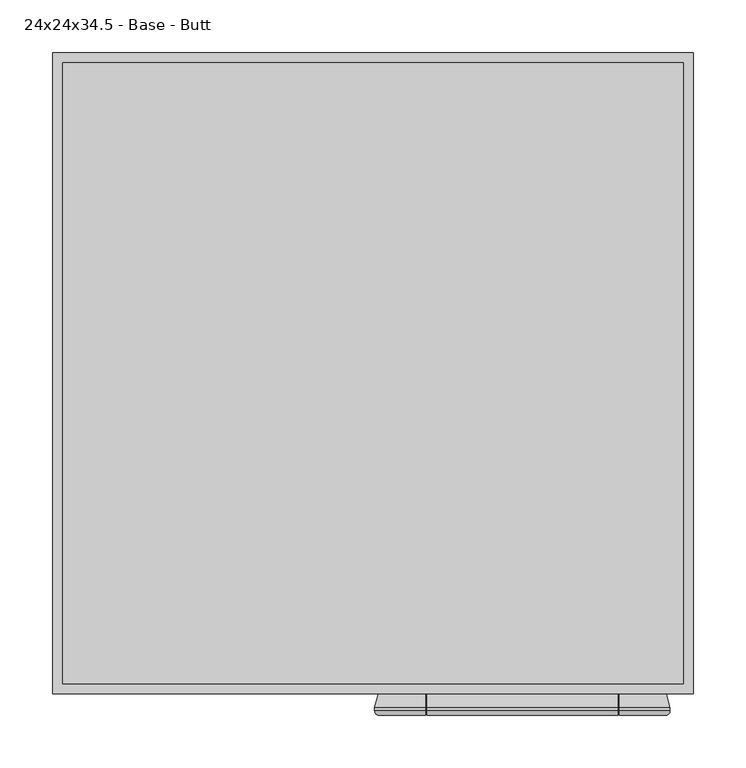
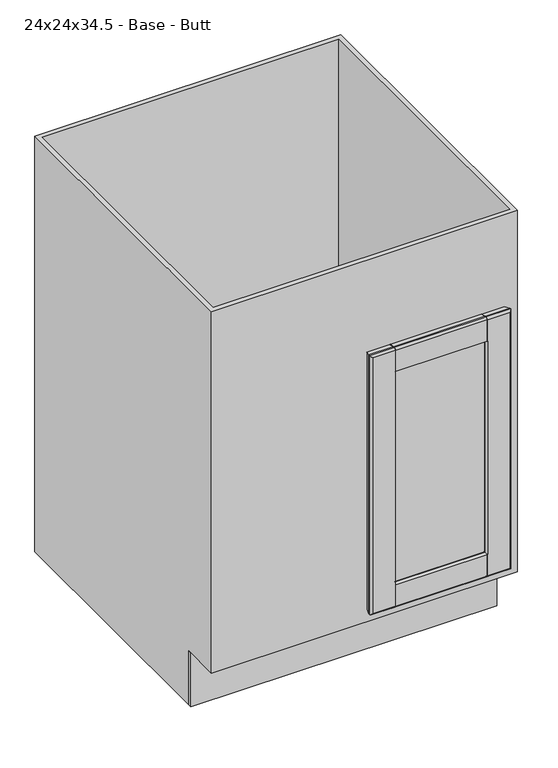
"""IFC4 building model written with IfcOpenShell, lengths in millimetres: furniture geometry, Cabinet-Base-Merillat-Double_Door-Marlin : 24x24x34.5 - Base - Butt."""

from ifc_helpers import new_model, si_unit, frame, origin, origin_with_axes, place, context, project, spatial, polyline, circle_curve, ellipse_curve, outline, extrude, faceted_brep, source, transform, mapped, element, save
from ifc_brep_helpers import plane_surface, cylinder_surface, advanced_brep


def furniture_24x24x34_5_base_butt_70915ae6(model_context):
    return source(origin(), model_context, "Body", "SolidModel", [
        advanced_brep(
        [(301.3127049, -625.4496, 685.8), (298.2162124, -629.92, 682.7035075), (298.2162124, -629.92, 142.7964925), (301.3127049, -625.4496, 139.7), (301.3127049, -622.681, 139.7), (301.3127049, -622.681, 685.8), (297.8075049, -609.6, 143.2052), (297.8075049, -609.6, 682.2948), (253.1115422, -609.6, 637.5988372), (253.1115422, -609.6, 187.9011628), (252.7414105, -610.39375, 188.2712945), (250.6602514, -614.85681, 190.3524535), (250.6602514, -614.85681, 635.1475465), (252.7414105, -610.39375, 637.2287055), (252.0600209, -617.0969093, 188.952684), (252.0600209, -617.0969093, 636.547316), (266.3877049, -617.347, 174.625), (266.3877049, -617.347, 650.875), (266.3877049, -622.173, 174.625), (266.3877049, -622.173, 650.875), (252.0600209, -622.4230907, 188.952684), (252.0600209, -622.4230907, 636.547316), (250.6602514, -624.66319, 190.3524535), (250.6602514, -624.66319, 635.1475465), (252.7414105, -629.12625, 188.2712945), (253.1086747, -629.9138508, 187.9040302), (253.1115422, -629.92, 637.5988372), (252.7414105, -629.12625, 637.2287055), (253.1086747, -629.92, 142.7964925), (253.1086747, -625.4496, 139.7), (23.4216974, -629.92, 142.7964925), (20.3252049, -625.4496, 139.7), (68.4894236, -625.4496, 139.7), (68.4894236, -629.92, 142.7964925), (251.5211747, -625.4496, 139.7), (251.5211747, -629.92, 142.7964925), (70.0769236, -629.92, 142.7964925), (70.0769236, -625.4496, 139.7), (253.1086747, -622.681, 139.7), (20.3252049, -622.681, 139.7), (68.4894236, -622.681, 139.7), (251.5211747, -622.681, 139.7), (70.0769236, -622.681, 139.7), (253.1086747, -609.6, 143.2052), (23.8304049, -609.6, 143.2052), (68.4894236, -609.6, 143.2052), (251.5211747, -609.6, 143.2052), (70.0769236, -609.6, 143.2052), (70.9776584, -614.85681, 190.3524535), (251.5211747, -610.39375, 188.2712945), (251.5211747, -609.6, 187.9011628), (70.0769236, -609.6, 187.9011628), (70.0769236, -610.39375, 188.2712945), (68.8964994, -610.39375, 188.2712945), (69.577889, -617.0969093, 188.952684), (55.2502049, -617.347, 174.625), (55.2502049, -622.173, 174.625), (69.577889, -622.4230907, 188.952684), (70.9776584, -624.66319, 190.3524535), (68.8964994, -629.12625, 188.2712945), (70.0769236, -629.12625, 188.2712945), (70.0769236, -629.92, 187.9011628), (251.5211747, -629.92, 187.9011628), (251.5211747, -629.12625, 188.2712945), (23.4216974, -629.92, 682.7035075), (20.3252049, -625.4496, 685.8), (20.3252049, -622.681, 685.8), (23.8304049, -609.6, 682.2948), (68.5263677, -609.6, 187.9011628), (68.5263677, -609.6, 637.5988372), (68.8964994, -610.39375, 637.2287055), (70.9776584, -614.85681, 635.1475465), (69.577889, -617.0969093, 636.547316), (55.2502049, -617.347, 650.875), (55.2502049, -622.173, 650.875), (69.577889, -622.4230907, 636.547316), (70.9776584, -624.66319, 635.1475465), (68.8964994, -629.12625, 637.2287055), (68.5263677, -629.92, 637.5988372), (68.5263677, -629.92, 187.9011628), (68.4894236, -629.92, 682.7035075), (68.4894236, -625.4496, 685.8), (253.1086747, -625.4496, 685.8), (253.1086747, -629.92, 682.7035075), (70.0769236, -625.4496, 685.8), (70.0769236, -629.92, 682.7035075), (251.5211747, -629.92, 682.7035075), (251.5211747, -625.4496, 685.8), (68.4894236, -622.681, 685.8), (253.1086747, -622.681, 685.8), (70.0769236, -622.681, 685.8), (251.5211747, -622.681, 685.8), (68.4894236, -609.6, 682.2948), (253.1086747, -609.6, 682.2948), (70.0769236, -609.6, 682.2948), (251.5211747, -609.6, 682.2948), (70.0769236, -609.6, 637.5988372), (251.5211747, -609.6, 637.5988372), (70.0769236, -610.39375, 637.2287055), (251.5211747, -610.39375, 637.2287055), (251.5211747, -629.12625, 637.2287055), (251.5211747, -629.92, 637.5988372), (70.0769236, -629.92, 637.5988372), (70.0769236, -629.12625, 637.2287055), (70.0769236, -610.39375, 681.6857412), (70.0769236, -622.7855037, 685.00625), (70.0769236, -625.4496, 685.00625), (70.0769236, -629.12625, 682.5526052), (68.4894236, -629.12625, 637.2287055), (68.4894236, -629.12625, 682.5526052), (68.4894236, -625.4496, 685.00625), (68.4894236, -622.7855037, 685.00625), (68.4894236, -610.39375, 681.6857412), (68.4894236, -610.39375, 637.2287055), (253.1086747, -610.39375, 637.2287055), (253.1086747, -610.39375, 681.6857412), (253.1086747, -622.7855037, 685.00625), (253.1086747, -625.4496, 685.00625), (253.1086747, -629.12625, 682.5526052), (253.1086747, -629.12625, 637.2287055), (251.5211747, -629.12625, 682.5526052), (251.5211747, -625.4496, 685.00625), (251.5211747, -622.7855037, 685.00625), (251.5211747, -610.39375, 681.6857412), (253.1086747, -629.12625, 188.2712945), (253.1086747, -629.12625, 142.9473948), (253.1086747, -625.4496, 140.49375), (253.1086747, -622.7855037, 140.49375), (253.1086747, -610.39375, 143.8142588), (253.1086747, -610.39375, 188.2712945), (251.5211747, -610.39375, 143.8142588), (251.5211747, -622.7855037, 140.49375), (251.5211747, -625.4496, 140.49375), (251.5211747, -629.12625, 142.9473948), (70.0769236, -629.12625, 142.9473948), (70.0769236, -625.4496, 140.49375), (70.0769236, -622.7855037, 140.49375), (70.0769236, -610.39375, 143.8142588), (68.4894236, -629.12625, 188.2712945), (68.4894236, -610.39375, 188.2712945), (68.4894236, -610.39375, 143.8142588), (68.4894236, -622.7855037, 140.49375), (68.4894236, -625.4496, 140.49375), (68.4894236, -629.12625, 142.9473948)],
        [
            (0, 1, ellipse_curve(frame((296.5375049, -625.4496, 681.0248), z_axis=(0.7071067811865475, 0.0, -0.7071067811865475), x_axis=(0.7071067811865474, 0.0, 0.7071067811865476)), 6.7531526, 4.7752)),
            (1, 2),
            (2, 3, ellipse_curve(frame((296.5375049, -625.4496, 144.4752), z_axis=(0.7071067811865475, 0.0, 0.7071067811865475), x_axis=(-0.7071067811865474, 0.0, 0.7071067811865476)), 6.7531526, 4.7752)),
            (3, 0),
            (3, 4),
            (4, 5),
            (5, 0),
            (4, 6),
            (6, 7),
            (7, 5),
            (8, 9),
            (9, 10),
            (10, 11),
            (11, 12),
            (12, 13),
            (13, 8),
            (11, 14, ellipse_curve(frame((252.0875049, -615.5223492, 188.9252), z_axis=(0.7071067811865475, 0.0, 0.7071067811865475), x_axis=(-0.7071067811865474, 0.0, 0.7071067811865476)), 2.2271035, 1.5748)),
            (14, 15),
            (15, 12, ellipse_curve(frame((252.0875049, -615.5223492, 636.5748), z_axis=(0.7071067811865475, 0.0, -0.7071067811865475), x_axis=(0.7071067811865474, 0.0, 0.7071067811865476)), 2.2271035, 1.5748)),
            (14, 16),
            (16, 17),
            (17, 15),
            (16, 18),
            (18, 19),
            (19, 17),
            (18, 20),
            (20, 21),
            (21, 19),
            (20, 22, ellipse_curve(frame((252.0875049, -623.9976508, 188.9252), z_axis=(0.7071067811865475, 0.0, 0.7071067811865475), x_axis=(-0.7071067811865474, 0.0, 0.7071067811865476)), 2.2271035, 1.5748)),
            (22, 23),
            (23, 21, ellipse_curve(frame((252.0875049, -623.9976508, 636.5748), z_axis=(0.7071067811865475, 0.0, -0.7071067811865475), x_axis=(0.7071067811865474, 0.0, 0.7071067811865476)), 2.2271035, 1.5748)),
            (22, 24),
            (24, 25),
            (25, 26),
            (26, 27),
            (27, 23),
            (2, 28),
            (28, 29, circle_curve(frame((253.1086747, -625.4496, 144.4752), z_axis=(1.0, 0.0, 0.0), x_axis=(0.0, 1.0, 0.0)), 4.7752)),
            (29, 3),
            (30, 31, ellipse_curve(frame((25.1004049, -625.4496, 144.4752), z_axis=(0.7071067811865475, 0.0, -0.7071067811865475), x_axis=(0.7071067811865476, 0.0, 0.7071067811865474)), 6.7531526, 4.7752)),
            (31, 32),
            (32, 33, circle_curve(frame((68.4894236, -625.4496, 144.4752), z_axis=(-1.0, 0.0, 0.0), x_axis=(0.0, 1.0, 0.0)), 4.7752)),
            (33, 30),
            (34, 35, circle_curve(frame((251.5211747, -625.4496, 144.4752), z_axis=(-1.0, 0.0, 0.0), x_axis=(0.0, 1.0, 0.0)), 4.7752)),
            (35, 36),
            (36, 37, circle_curve(frame((70.0769236, -625.4496, 144.4752), z_axis=(1.0, 0.0, 0.0), x_axis=(0.0, 1.0, 0.0)), 4.7752)),
            (37, 34),
            (29, 38),
            (38, 4),
            (31, 39),
            (39, 40),
            (40, 32),
            (41, 34),
            (37, 42),
            (42, 41),
            (38, 43),
            (43, 6),
            (39, 44),
            (44, 45),
            (45, 40),
            (46, 41),
            (42, 47),
            (47, 46),
            (48, 11),
            (10, 49),
            (49, 50),
            (50, 51),
            (51, 52),
            (52, 53),
            (53, 48),
            (48, 54, ellipse_curve(frame((69.5504049, -615.5223492, 188.9252), z_axis=(0.7071067811865475, 0.0, -0.7071067811865475), x_axis=(0.7071067811865476, 0.0, 0.7071067811865474)), 2.2271035, 1.5748)),
            (54, 14),
            (54, 55),
            (55, 16),
            (55, 56),
            (56, 18),
            (56, 57),
            (57, 20),
            (57, 58, ellipse_curve(frame((69.5504049, -623.9976508, 188.9252), z_axis=(0.7071067811865475, 0.0, -0.7071067811865475), x_axis=(0.7071067811865476, 0.0, 0.7071067811865474)), 2.2271035, 1.5748)),
            (58, 22),
            (58, 59),
            (59, 60),
            (60, 61),
            (61, 62),
            (62, 63),
            (63, 24),
            (30, 64),
            (64, 65, ellipse_curve(frame((25.1004049, -625.4496, 681.0248), z_axis=(-0.7071067811865475, 0.0, -0.7071067811865475), x_axis=(0.7071067811865474, 0.0, -0.7071067811865476)), 6.7531526, 4.7752)),
            (65, 31),
            (65, 66),
            (66, 39),
            (66, 67),
            (67, 44),
            (68, 69),
            (69, 70),
            (70, 71),
            (71, 48),
            (53, 68),
            (71, 72, ellipse_curve(frame((69.5504049, -615.5223492, 636.5748), z_axis=(-0.7071067811865475, 0.0, -0.7071067811865475), x_axis=(0.7071067811865474, 0.0, -0.7071067811865476)), 2.2271035, 1.5748)),
            (72, 54),
            (72, 73),
            (73, 55),
            (73, 74),
            (74, 56),
            (74, 75),
            (75, 57),
            (75, 76, ellipse_curve(frame((69.5504049, -623.9976508, 636.5748), z_axis=(-0.7071067811865475, 0.0, -0.7071067811865475), x_axis=(0.7071067811865474, 0.0, -0.7071067811865476)), 2.2271035, 1.5748)),
            (76, 58),
            (76, 77),
            (77, 78),
            (78, 79),
            (79, 59),
            (64, 80),
            (80, 81, circle_curve(frame((68.4894236, -625.4496, 681.0248), z_axis=(-1.0, 0.0, 0.0), x_axis=(0.0, 1.0, 0.0)), 4.7752)),
            (81, 65),
            (0, 82),
            (82, 83, circle_curve(frame((253.1086747, -625.4496, 681.0248), z_axis=(1.0, 0.0, 0.0), x_axis=(0.0, 1.0, 0.0)), 4.7752)),
            (83, 1),
            (84, 85, circle_curve(frame((70.0769236, -625.4496, 681.0248), z_axis=(1.0, 0.0, 0.0), x_axis=(0.0, 1.0, 0.0)), 4.7752)),
            (85, 86),
            (86, 87, circle_curve(frame((251.5211747, -625.4496, 681.0248), z_axis=(-1.0, 0.0, 0.0), x_axis=(0.0, 1.0, 0.0)), 4.7752)),
            (87, 84),
            (81, 88),
            (88, 66),
            (5, 89),
            (89, 82),
            (90, 84),
            (87, 91),
            (91, 90),
            (88, 92),
            (92, 67),
            (7, 93),
            (93, 89),
            (94, 90),
            (91, 95),
            (95, 94),
            (43, 9),
            (8, 93),
            (92, 69),
            (68, 45),
            (96, 94),
            (95, 97),
            (97, 96),
            (50, 46),
            (47, 51),
            (12, 71),
            (70, 98),
            (98, 96),
            (97, 99),
            (99, 13),
            (15, 72),
            (17, 73),
            (19, 74),
            (21, 75),
            (23, 76),
            (27, 100),
            (100, 101),
            (101, 102),
            (102, 103),
            (103, 77),
            (83, 26),
            (25, 28),
            (33, 79),
            (78, 80),
            (85, 102),
            (101, 86),
            (35, 62),
            (61, 36),
            (98, 104),
            (104, 105),
            (105, 106),
            (106, 107, circle_curve(frame((70.0769236, -625.4496, 681.0248), z_axis=(1.0, 0.0, 0.0), x_axis=(0.0, 0.0, 1.0)), 3.98145)),
            (107, 103),
            (78, 108),
            (108, 109),
            (109, 110, circle_curve(frame((68.4894236, -625.4496, 681.0248), z_axis=(-1.0, 0.0, 0.0), x_axis=(0.0, 0.0, 1.0)), 3.98145)),
            (110, 111),
            (111, 112),
            (112, 113),
            (113, 69),
            (77, 108),
            (107, 109),
            (106, 110),
            (105, 111),
            (104, 112),
            (70, 113),
            (8, 114),
            (114, 115),
            (115, 116),
            (116, 117),
            (117, 118, circle_curve(frame((253.1086747, -625.4496, 681.0248), z_axis=(1.0, 0.0, 0.0), x_axis=(0.0, 0.0, 1.0)), 3.98145)),
            (118, 119),
            (119, 26),
            (100, 120),
            (120, 121, circle_curve(frame((251.5211747, -625.4496, 681.0248), z_axis=(-1.0, 0.0, 0.0), x_axis=(0.0, 0.0, 1.0)), 3.98145)),
            (121, 122),
            (122, 123),
            (123, 99),
            (119, 27),
            (118, 120),
            (117, 121),
            (116, 122),
            (115, 123),
            (114, 13),
            (25, 124),
            (124, 125),
            (125, 126, circle_curve(frame((253.1086747, -625.4496, 144.4752), z_axis=(1.0, 0.0, 0.0), x_axis=(0.0, 0.0, 1.0)), 3.98145)),
            (126, 127),
            (127, 128),
            (128, 129),
            (129, 9),
            (49, 130),
            (130, 131),
            (131, 132),
            (132, 133, circle_curve(frame((251.5211747, -625.4496, 144.4752), z_axis=(-1.0, 0.0, 0.0), x_axis=(0.0, 0.0, 1.0)), 3.98145)),
            (133, 63),
            (129, 10),
            (128, 130),
            (127, 131),
            (126, 132),
            (125, 133),
            (124, 24),
            (60, 134),
            (134, 135, circle_curve(frame((70.0769236, -625.4496, 144.4752), z_axis=(1.0, 0.0, 0.0), x_axis=(0.0, 0.0, 1.0)), 3.98145)),
            (135, 136),
            (136, 137),
            (137, 52),
            (138, 79),
            (68, 139),
            (139, 140),
            (140, 141),
            (141, 142),
            (142, 143, circle_curve(frame((68.4894236, -625.4496, 144.4752), z_axis=(-1.0, 0.0, 0.0), x_axis=(0.0, 0.0, 1.0)), 3.98145)),
            (143, 138),
            (138, 59),
            (53, 139),
            (137, 140),
            (136, 141),
            (135, 142),
            (134, 143),
        ],
        [
            cylinder_surface(frame((296.5375049, -625.4496, 685.8), z_axis=(0.0, 0.0, 1.0), x_axis=(0.0, 1.0, 0.0)), 4.7752),
            plane_surface(frame((301.3127049, -625.4496, 685.8), z_axis=(1.0, 0.0, 0.0), x_axis=(0.0, 0.0, -1.0))),
            plane_surface(frame((301.3127049, -622.681, 685.8), z_axis=(0.9659229350723619, 0.25882983502910506, 0.0), x_axis=(0.0, 0.0, -1.0))),
            plane_surface(frame((253.1115422, -609.6, 637.5988372), z_axis=(-0.9063077870366099, 0.4226182617407856, 0.0), x_axis=(0.0, 0.0, -1.0))),
            cylinder_surface(frame((252.0875049, -615.5223492, 685.8), z_axis=(0.0, 0.0, 1.0000000000000002), x_axis=(-0.01745240643729364, -0.9998476951563912, 0.0)), 1.5748),
            plane_surface(frame((252.0600209, -617.0969093, 636.547316), z_axis=(-0.017452406437322144, -0.9998476951563906, 0.0), x_axis=(0.0, 0.0, -1.0))),
            plane_surface(frame((266.3877049, -617.347, 650.875), z_axis=(-1.0, 0.0, 0.0), x_axis=(0.0, 0.0, -1.0))),
            plane_surface(frame((266.3877049, -622.173, 650.875), z_axis=(-0.01745240643727848, 0.9998476951563914, 0.0), x_axis=(0.0, 0.0, -1.0))),
            cylinder_surface(frame((252.0875049, -623.9976508, 685.8), z_axis=(0.0, 0.0, 1.0000000000000002), x_axis=(-0.9063077870367326, -0.42261826174052236, 0.0)), 1.5748),
            plane_surface(frame((250.6602514, -624.66319, 635.1475465), z_axis=(-0.9063077870366333, -0.4226182617407352, 0.0), x_axis=(0.0, 0.0, -1.0))),
            cylinder_surface(frame((301.3127049, -625.4496, 144.4752), z_axis=(1.0, 0.0, 0.0), x_axis=(0.0, 1.0, 0.0)), 4.7752),
            plane_surface(frame((301.3127049, -625.4496, 139.7), z_axis=(0.0, 0.0, -1.0), x_axis=(-1.0, 0.0, 0.0))),
            plane_surface(frame((301.3127049, -622.681, 139.7), z_axis=(0.0, 0.25882983502910506, -0.9659229350723619), x_axis=(-1.0, 0.0, 0.0))),
            plane_surface(frame((253.1115422, -609.6, 187.9011628), z_axis=(0.0, 0.4226182617407856, 0.9063077870366099), x_axis=(-1.0, 0.0, 0.0))),
            cylinder_surface(frame((301.3127049, -615.5223492, 188.9252), z_axis=(1.0000000000000002, 0.0, 0.0), x_axis=(0.0, -0.9998476951563912, 0.01745240643729364)), 1.5748),
            plane_surface(frame((252.0600209, -617.0969093, 188.952684), z_axis=(0.0, -0.9998476951563906, 0.017452406437322144), x_axis=(-1.0, 0.0, 0.0))),
            plane_surface(frame((266.3877049, -617.347, 174.625), z_axis=(0.0, 0.0, 1.0), x_axis=(-1.0, 0.0, 0.0))),
            plane_surface(frame((266.3877049, -622.173, 174.625), z_axis=(0.0, 0.9998476951563914, 0.01745240643727848), x_axis=(-1.0, 0.0, 0.0))),
            cylinder_surface(frame((301.3127049, -623.9976508, 188.9252), z_axis=(1.0000000000000002, 0.0, 0.0), x_axis=(0.0, -0.42261826174052236, 0.9063077870367326)), 1.5748),
            plane_surface(frame((250.6602514, -624.66319, 190.3524535), z_axis=(0.0, -0.4226182617407352, 0.9063077870366333), x_axis=(-1.0, 0.0, 0.0))),
            cylinder_surface(frame((25.1004049, -625.4496, 139.7), z_axis=(0.0, 0.0, -1.0), x_axis=(0.0, 1.0, 0.0)), 4.7752),
            plane_surface(frame((20.3252049, -625.4496, 139.7), z_axis=(-1.0, 0.0, 0.0), x_axis=(0.0, 0.0, 1.0))),
            plane_surface(frame((20.3252049, -622.681, 139.7), z_axis=(-0.9659229350723619, 0.25882983502910506, 0.0), x_axis=(0.0, 0.0, 1.0))),
            plane_surface(frame((68.5263677, -609.6, 187.9011628), z_axis=(0.9063077870366099, 0.4226182617407856, 0.0), x_axis=(0.0, 0.0, 1.0))),
            cylinder_surface(frame((69.5504049, -615.5223492, 139.7), z_axis=(0.0, 0.0, -1.0000000000000002), x_axis=(0.01745240643729364, -0.9998476951563912, 0.0)), 1.5748),
            plane_surface(frame((69.577889, -617.0969093, 188.952684), z_axis=(0.017452406437322144, -0.9998476951563906, 0.0), x_axis=(0.0, 0.0, 1.0))),
            plane_surface(frame((55.2502049, -617.347, 174.625), z_axis=(1.0, 0.0, 0.0), x_axis=(0.0, 0.0, 1.0))),
            plane_surface(frame((55.2502049, -622.173, 174.625), z_axis=(0.01745240643727848, 0.9998476951563914, 0.0), x_axis=(0.0, 0.0, 1.0))),
            cylinder_surface(frame((69.5504049, -623.9976508, 139.7), z_axis=(0.0, 0.0, -1.0000000000000002), x_axis=(0.9063077870367326, -0.42261826174052236, 0.0)), 1.5748),
            plane_surface(frame((70.9776584, -624.66319, 190.3524535), z_axis=(0.9063077870366333, -0.4226182617407352, 0.0), x_axis=(0.0, 0.0, 1.0))),
            cylinder_surface(frame((20.3252049, -625.4496, 681.0248), z_axis=(-1.0, 0.0, 0.0), x_axis=(0.0, 1.0, 0.0)), 4.7752),
            plane_surface(frame((20.3252049, -625.4496, 685.8), z_axis=(0.0, 0.0, 1.0), x_axis=(1.0, 0.0, 0.0))),
            plane_surface(frame((20.3252049, -622.681, 685.8), z_axis=(0.0, 0.25882983502910506, 0.9659229350723619), x_axis=(1.0, 0.0, 0.0))),
            plane_surface(frame((23.8304049, -609.6, 682.2948), z_axis=(0.0, 1.0, 0.0), x_axis=(1.0, 0.0, 0.0))),
            plane_surface(frame((68.5263677, -609.6, 637.5988372), z_axis=(0.0, 0.4226182617407856, -0.9063077870366099), x_axis=(1.0, 0.0, 0.0))),
            cylinder_surface(frame((20.3252049, -615.5223492, 636.5748), z_axis=(-1.0000000000000002, 0.0, 0.0), x_axis=(0.0, -0.9998476951563912, -0.01745240643729364)), 1.5748),
            plane_surface(frame((69.577889, -617.0969093, 636.547316), z_axis=(0.0, -0.9998476951563906, -0.017452406437322144), x_axis=(1.0, 0.0, 0.0))),
            plane_surface(frame((55.2502049, -617.347, 650.875), z_axis=(0.0, 0.0, -1.0), x_axis=(1.0, 0.0, 0.0))),
            plane_surface(frame((55.2502049, -622.173, 650.875), z_axis=(0.0, 0.9998476951563914, -0.01745240643727848), x_axis=(1.0, 0.0, 0.0))),
            cylinder_surface(frame((20.3252049, -623.9976508, 636.5748), z_axis=(-1.0000000000000002, 0.0, 0.0), x_axis=(0.0, -0.42261826174052236, -0.9063077870367326)), 1.5748),
            plane_surface(frame((70.9776584, -624.66319, 635.1475465), z_axis=(0.0, -0.4226182617407352, -0.9063077870366333), x_axis=(1.0, 0.0, 0.0))),
            plane_surface(frame((68.5263677, -629.92, 637.5988372), z_axis=(0.0, -1.0, 0.0), x_axis=(1.0, 0.0, 0.0))),
            plane_surface(frame((70.0769236, -629.92, 637.5988372), z_axis=(-1.0, 0.0, 0.0), x_axis=(0.0, 0.906307787036771, -0.4226182617404399))),
            plane_surface(frame((68.4894236, -629.92, 637.5988372), z_axis=(1.0, 0.0, 0.0), x_axis=(0.0, -0.906307787036771, 0.4226182617404399))),
            plane_surface(frame((70.0769236, -629.92, 637.5988372), z_axis=(0.0, 0.4226182617404399, 0.906307787036771), x_axis=(-1.0, 0.0, 0.0))),
            plane_surface(frame((70.0769236, -629.12625, 637.2287055), z_axis=(0.0, -1.0, 0.0), x_axis=(-1.0, 0.0, 0.0))),
            cylinder_surface(frame((68.4894236, -625.4496, 681.0248), z_axis=(-1.0, 0.0, 0.0), x_axis=(0.0, 0.0, 1.0)), 3.98145),
            plane_surface(frame((70.0769236, -625.4496, 685.00625), z_axis=(0.0, 0.0, 1.0), x_axis=(-1.0, 0.0, 0.0))),
            plane_surface(frame((70.0769236, -622.7855037, 685.00625), z_axis=(0.0, 0.25882983502913415, 0.9659229350723542), x_axis=(-1.0, 0.0, 0.0))),
            plane_surface(frame((70.0769236, -610.39375, 681.6857412), z_axis=(0.0, 1.0, 0.0), x_axis=(-1.0, 0.0, 0.0))),
            plane_surface(frame((70.0769236, -610.39375, 637.2287055), z_axis=(0.0, -0.4226182617405111, 0.9063077870367379), x_axis=(-1.0, 0.0, 0.0))),
            plane_surface(frame((253.1086747, -629.92, 637.5988372), z_axis=(-1.0, 0.0, 0.0), x_axis=(0.0, 0.9063077870367783, -0.42261826174042444))),
            plane_surface(frame((251.5211747, -629.92, 637.5988372), z_axis=(1.0, 0.0, 0.0), x_axis=(0.0, -0.9063077870367783, 0.42261826174042444))),
            plane_surface(frame((253.1086747, -629.92, 637.5988372), z_axis=(0.0, 0.42261826174042444, 0.9063077870367783), x_axis=(-1.0, 0.0, 0.0))),
            plane_surface(frame((253.1086747, -629.12625, 637.2287055), z_axis=(0.0, -1.0, 0.0), x_axis=(-1.0, 0.0, 0.0))),
            cylinder_surface(frame((251.5211747, -625.4496, 681.0248), z_axis=(-1.0, 0.0, 0.0), x_axis=(0.0, 0.0, 1.0)), 3.98145),
            plane_surface(frame((253.1086747, -625.4496, 685.00625), z_axis=(0.0, 0.0, 1.0), x_axis=(-1.0, 0.0, 0.0))),
            plane_surface(frame((253.1086747, -622.7855037, 685.00625), z_axis=(0.0, 0.25882983502911566, 0.965922935072359), x_axis=(-1.0, 0.0, 0.0))),
            plane_surface(frame((253.1086747, -610.39375, 681.6857412), z_axis=(0.0, 1.0, 0.0), x_axis=(-1.0, 0.0, 0.0))),
            plane_surface(frame((253.1086747, -610.39375, 637.2287055), z_axis=(0.0, -0.42261826174056427, 0.9063077870367131), x_axis=(-1.0, 0.0, 0.0))),
            plane_surface(frame((253.1086747, -625.4496, 149.2504), z_axis=(-1.0, 0.0, 0.0), x_axis=(0.0, -1.0, 0.0))),
            plane_surface(frame((251.5211747, -625.4496, 149.2504), z_axis=(1.0, 0.0, 0.0), x_axis=(0.0, 1.0, 0.0))),
            plane_surface(frame((253.1086747, -609.6, 187.9011628), z_axis=(0.0, -0.42261826173999295, -0.9063077870369795), x_axis=(-1.0, 0.0, 0.0))),
            plane_surface(frame((253.1086747, -610.39375, 188.2712945), z_axis=(0.0, 1.0, 0.0), x_axis=(-1.0, 0.0, 0.0))),
            plane_surface(frame((253.1086747, -610.39375, 143.8142588), z_axis=(0.0, 0.2588298350290845, -0.9659229350723675), x_axis=(-1.0, 0.0, 0.0))),
            plane_surface(frame((253.1086747, -622.7855037, 140.49375), z_axis=(0.0, 0.0, -1.0), x_axis=(-1.0, 0.0, 0.0))),
            cylinder_surface(frame((251.5211747, -625.4496, 144.4752), z_axis=(-1.0, 0.0, 0.0), x_axis=(0.0, 0.0, 1.0)), 3.98145),
            plane_surface(frame((253.1086747, -629.12625, 142.9473948), z_axis=(0.0, -1.0, 0.0), x_axis=(-1.0, 0.0, 0.0))),
            plane_surface(frame((253.1086747, -629.12625, 188.2712945), z_axis=(0.0, 0.4226182617407698, -0.9063077870366172), x_axis=(-1.0, 0.0, 0.0))),
            plane_surface(frame((70.0769236, -629.12625, 188.2712945), z_axis=(-1.0, 0.0, 0.0), x_axis=(0.0, -0.906307787036583, -0.42261826174084305))),
            plane_surface(frame((68.4894236, -629.12625, 188.2712945), z_axis=(1.0, 0.0, 0.0), x_axis=(0.0, 0.906307787036583, 0.42261826174084305))),
            plane_surface(frame((70.0769236, -629.12625, 188.2712945), z_axis=(0.0, 0.42261826174084305, -0.906307787036583), x_axis=(-1.0, 0.0, 0.0))),
            plane_surface(frame((70.0769236, -609.6, 187.9011628), z_axis=(0.0, -0.42261826174073325, -0.9063077870366342), x_axis=(-1.0, 0.0, 0.0))),
            plane_surface(frame((70.0769236, -610.39375, 188.2712945), z_axis=(0.0, 1.0, 0.0), x_axis=(-1.0, 0.0, 0.0))),
            plane_surface(frame((70.0769236, -610.39375, 143.8142588), z_axis=(0.0, 0.2588298350290967, -0.9659229350723642), x_axis=(-1.0, 0.0, 0.0))),
            plane_surface(frame((70.0769236, -622.7855037, 140.49375), z_axis=(0.0, 0.0, -1.0), x_axis=(-1.0, 0.0, 0.0))),
            cylinder_surface(frame((68.4894236, -625.4496, 144.4752), z_axis=(-1.0, 0.0, 0.0), x_axis=(0.0, 0.0, 1.0)), 3.98145),
            plane_surface(frame((70.0769236, -629.12625, 142.9473948), z_axis=(0.0, -1.0, 0.0), x_axis=(-1.0, 0.0, 0.0))),
        ],
        [
            (0, [[1, 2, 3, 4]]),
            (1, [[-4, 5, 6, 7]]),
            (2, [[-6, 8, 9, 10]]),
            (3, [[11, 12, 13, 14, 15, 16]]),
            (4, [[-14, 17, 18, 19]]),
            (5, [[-18, 20, 21, 22]]),
            (6, [[-21, 23, 24, 25]]),
            (7, [[-24, 26, 27, 28]]),
            (8, [[-27, 29, 30, 31]]),
            (9, [[-30, 32, 33, 34, 35, 36]]),
            (10, [[-3, 37, 38, 39]]),
            (10, [[40, 41, 42, 43]]),
            (10, [[44, 45, 46, 47]]),
            (11, [[-5, -39, 48, 49]]),
            (11, [[50, 51, 52, -41]]),
            (11, [[53, -47, 54, 55]]),
            (12, [[-8, -49, 56, 57]]),
            (12, [[58, 59, 60, -51]]),
            (12, [[61, -55, 62, 63]]),
            (13, [[64, -13, 65, 66, 67, 68, 69, 70]]),
            (14, [[-17, -64, 71, 72]]),
            (15, [[-20, -72, 73, 74]]),
            (16, [[-23, -74, 75, 76]]),
            (17, [[-26, -76, 77, 78]]),
            (18, [[-29, -78, 79, 80]]),
            (19, [[-80, 81, 82, 83, 84, 85, 86, -32]]),
            (20, [[-40, 87, 88, 89]]),
            (21, [[-50, -89, 90, 91]]),
            (22, [[-58, -91, 92, 93]]),
            (23, [[94, 95, 96, 97, -70, 98]]),
            (24, [[-71, -97, 99, 100]]),
            (25, [[-73, -100, 101, 102]]),
            (26, [[-75, -102, 103, 104]]),
            (27, [[-77, -104, 105, 106]]),
            (28, [[-79, -106, 107, 108]]),
            (29, [[-108, 109, 110, 111, 112, -81]]),
            (30, [[-88, 113, 114, 115]]),
            (30, [[-1, 116, 117, 118]]),
            (30, [[119, 120, 121, 122]]),
            (31, [[-90, -115, 123, 124]]),
            (31, [[-7, 125, 126, -116]]),
            (31, [[127, -122, 128, 129]]),
            (32, [[-92, -124, 130, 131]]),
            (32, [[-10, 132, 133, -125]]),
            (32, [[134, -129, 135, 136]]),
            (33, [[-9, -57, 137, -11, 138, -132]]),
            (33, [[-93, -131, 139, -94, 140, -59]]),
            (33, [[141, -136, 142, 143]]),
            (33, [[144, -63, 145, -67]]),
            (34, [[146, -96, 147, 148, -143, 149, 150, -15]]),
            (35, [[-19, 151, -99, -146]]),
            (36, [[-22, 152, -101, -151]]),
            (37, [[-25, 153, -103, -152]]),
            (38, [[-28, 154, -105, -153]]),
            (39, [[-31, 155, -107, -154]]),
            (40, [[-155, -36, 156, 157, 158, 159, 160, -109]]),
            (41, [[-2, -118, 161, -34, 162, -37]]),
            (41, [[-87, -43, 163, -111, 164, -113]]),
            (41, [[165, -158, 166, -120]]),
            (41, [[167, -84, 168, -45]]),
            (42, [[169, 170, 171, 172, 173, -159, -165, -119, -127, -134, -141, -148]]),
            (43, [[174, 175, 176, 177, 178, 179, 180, -139, -130, -123, -114, -164]]),
            (44, [[-174, -110, 181]]),
            (45, [[-173, 182, -175, -181, -160]]),
            (46, [[-172, 183, -176, -182]]),
            (47, [[-171, 184, -177, -183]]),
            (48, [[-170, 185, -178, -184]]),
            (49, [[-169, -147, 186, -179, -185]]),
            (50, [[-180, -186, -95]]),
            (51, [[187, 188, 189, 190, 191, 192, 193, -161, -117, -126, -133, -138]]),
            (52, [[194, 195, 196, 197, 198, -149, -142, -135, -128, -121, -166, -157]]),
            (53, [[-193, 199, -35]]),
            (54, [[-192, 200, -194, -156, -199]]),
            (55, [[-191, 201, -195, -200]]),
            (56, [[-190, 202, -196, -201]]),
            (57, [[-189, 203, -197, -202]]),
            (58, [[-188, 204, -150, -198, -203]]),
            (59, [[-187, -16, -204]]),
            (60, [[205, 206, 207, 208, 209, 210, 211, -137, -56, -48, -38, -162]]),
            (61, [[212, 213, 214, 215, 216, -85, -167, -44, -53, -61, -144, -66]]),
            (62, [[-211, 217, -12]]),
            (63, [[-210, 218, -212, -65, -217]]),
            (64, [[-209, 219, -213, -218]]),
            (65, [[-208, 220, -214, -219]]),
            (66, [[-207, 221, -215, -220]]),
            (67, [[-206, 222, -86, -216, -221]]),
            (68, [[-205, -33, -222]]),
            (69, [[223, 224, 225, 226, 227, -68, -145, -62, -54, -46, -168, -83]]),
            (70, [[228, -163, -42, -52, -60, -140, 229, 230, 231, 232, 233, 234]]),
            (71, [[-228, 235, -112]]),
            (72, [[-229, -98, 236]]),
            (73, [[-227, 237, -230, -236, -69]]),
            (74, [[-226, 238, -231, -237]]),
            (75, [[-225, 239, -232, -238]]),
            (76, [[-224, 240, -233, -239]]),
            (77, [[-223, -82, -235, -234, -240]]),
        ],
    ),
        extrude(outline(polyline([(55.2502049, -622.173), (55.2502049, -617.347), (266.3877049, -617.347), (266.3877049, -622.173), (55.2502049, -622.173)])), frame((0.0, 0.0, 174.625), z_axis=(0.0, 0.0, 1.0), x_axis=(1.0, 0.0, 0.0)), (0.0, 0.0, 1.0), 476.25),
        faceted_brep([(323.5377049, 0.0, 0.0), (323.5377049, -529.43125, 0.0), (314.0127049, -529.43125, 0.0), (314.0127049, -9.525, 0.0), (-276.5372951, -9.525, 0.0), (-276.5372951, -529.43125, 0.0), (-286.0622951, -529.43125, 0.0), (-286.0622951, 0.0, 0.0), (-286.0622951, 0.0, 876.3), (323.5377049, 0.0, 876.3), (-286.0622951, -529.43125, 114.3), (-286.0622951, -609.6, 114.3), (-286.0622951, -609.6, 876.3), (323.5377049, -609.6, 876.3), (323.5377049, -609.6, 114.3), (323.5377049, -529.43125, 114.3), (314.0127049, -529.43125, 114.3), (314.0127049, -9.525, 114.3), (314.0127049, -600.075, 876.3), (314.0127049, -9.525, 876.3), (314.0127049, -9.525, 123.825), (314.0127049, -600.075, 123.825), (-276.5372951, -9.525, 114.3), (-276.5372951, -529.43125, 114.3), (-276.5372951, -9.525, 876.3), (-276.5372951, -600.075, 876.3), (-276.5372951, -600.075, 123.825), (-276.5372951, -9.525, 123.825)], [[[0, 1, 2, 3, 4, 5, 6, 7]], [[0, 7, 8, 9]], [[7, 6, 10, 11, 12, 8]], [[1, 0, 9, 13, 14, 15]], [[3, 2, 16, 17]], [[18, 19, 20, 21]], [[5, 4, 22, 23]], [[24, 25, 26, 27]], [[4, 3, 17, 22]], [[19, 24, 27, 20]], [[9, 8, 12, 13], [19, 18, 25, 24]], [[14, 11, 10, 23, 22, 17, 16, 15]], [[13, 12, 11, 14]], [[25, 18, 21, 26]], [[6, 5, 23, 10]], [[2, 1, 15, 16]], [[21, 20, 27, 26]]]),
        extrude(outline(polyline([(323.5377049, -529.43125), (323.5377049, -538.95625), (-286.0622951, -538.95625), (-286.0622951, -529.43125), (323.5377049, -529.43125)])), origin_with_axes(), (0.0, 0.0, 1.0), 114.3),
    ])


if __name__ == "__main__":
    model = new_model("IFC4")
    model_context = context("Model", 3, world=origin())
    ifc_project = project(units=[si_unit("LENGTHUNIT", "METRE", prefix="MILLI")], contexts=[model_context])
    site = spatial("IfcSite", under=ifc_project)
    building = spatial("IfcBuilding", under=site)
    placement = place(None, origin())
    furniture_24x24x34_5_base_butt_shape = furniture_24x24x34_5_base_butt_70915ae6(model_context)
    element("IfcFurniture", 1, ObjectType="Cabinet-Base-Merillat-Double_Door-Marlin : 24x24x34.5 - Base - Butt", at=placement, inside=building, context=model_context, shape_type="MappedRepresentation", body=[
        mapped(furniture_24x24x34_5_base_butt_shape, transform((0.0, 0.0, 0.0), x_axis=(1.0, 0.0, 0.0), y_axis=(0.0, 1.0, 0.0), z_axis=(0.0, 0.0, 1.0))),
    ])
    save(model, "model.ifc")

# Revit data of these elements
# Type "Cabinet-Base-Merillat-Double_Door-Marlin : 24x24x34.5 - Base - Butt"
#   URL = "http://www.merillat.com"
#   Toe Kick Note = "Toe Kick Covering is not included. To be purchased Separately."
#   Product Line = "Express"
#   Product Page URL = "http://www.merillat.com//our-products/rooms/kitchen"
#   Product Group = "Base Cabinet"
#   Product Documentation Link = "http://merillatbusiness.com/customer-resources/product-line-resources/merillat-classic/"
#   Model = "B24B"
#   Manufacturer = "Merillat"
#   Finish = "Wood"
#   Description = "Base Butt Door"
#   Construction Type = "Deep Sink Base"
#   Cabinet Construction Note = "BUTT doors without a center frame stile, For tray or shelf option,  replace HDS with the option code of your choice,  When depth is reduced  to 12\" or 15\" drawer becomes false front"
#   Assembly Code = "C1030410"
#   Toe Kick Height = 0' - 4 1/2"
#   Toe Kick Depth = 0' - 2 25/32"
#   Top and Bottom Spacing = 0' - 1"
#   Side Spacing = 0' - 0 7/8"
#   Cabinet Shell = 0' - 0 3/8"
#   Door Spacing = 0' - 0 1/8"
#   Depth = 2' - 0"
#   Height = 2' - 10 1/2"
#   Width = 2' - 0"
#   Cabinet Drawer Width = 1' - 10 1/4"
#   Cabinet Drawer Height = 0' - 5 1/2"
#   Cabinet Drawer 2 Drawer Width = 0' - 11 1/16"
#   Cabinet Door Width = 0' - 11 1/16"
#   Cabinet Door Height = 1' - 9 1/2"
#   COBie.Type = no
#   Two Drawer = no
#   Elevation Swing Line = yes
#   Partial Overlay = yes
#   One Drawer = yes
#   Full Overlay = no
#   Butt Option = yes
#   Toe Kick Material = Wood - Merillat - Raw Particle Board
#   Door Drawer Material = Wood - Merillat - Pecan(1)
#   Cabinet Material = Wood - Merillat - Pecan(1)
#   Cabinet Drawer Style 2 Drawer = element 819256
#   Cabinet Drawer Style = element 819255
#   Cabinet Door Style = element 819254
# Element 1 (IfcFurniture, "Cabinet-Base-Merillat-Double_Door-Marlin : 24x24x34.5 - Base - Butt")
#   Materials on its faces: "Wood - Merillat - Pecan(1)", "Wood - Merillat - Raw Particle Board"
# Materials
#   "Wood - Merillat - Raw Particle Board": class "Plastic", colour RGB 80 80 80, transparency 0, Description = "Plastic Laminate - Navy", Cost = 0
#   "Wood - Merillat - Pecan(1)": class "Wood", colour RGB 108 67 43, transparency 0, Cost = 0
